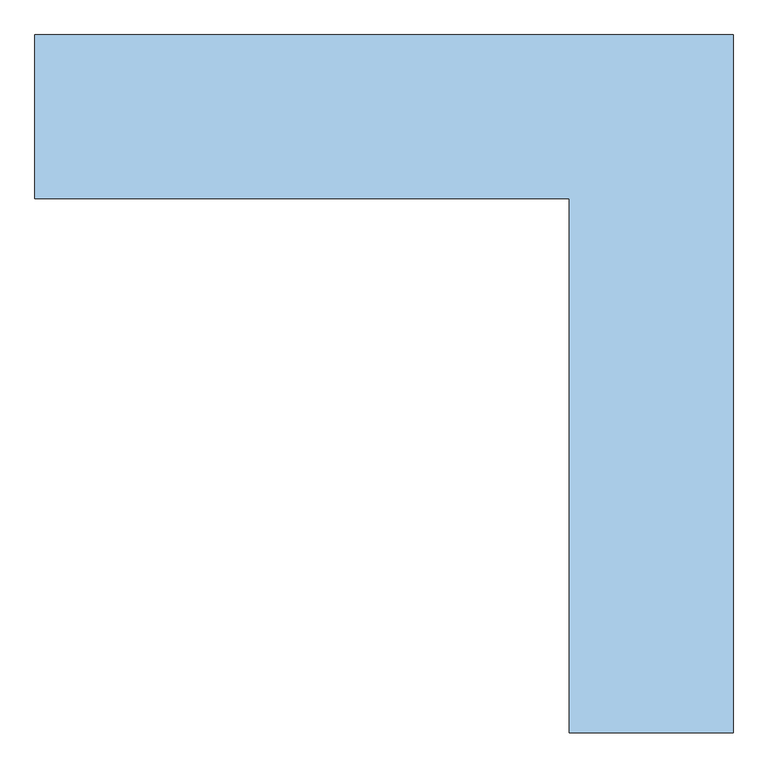
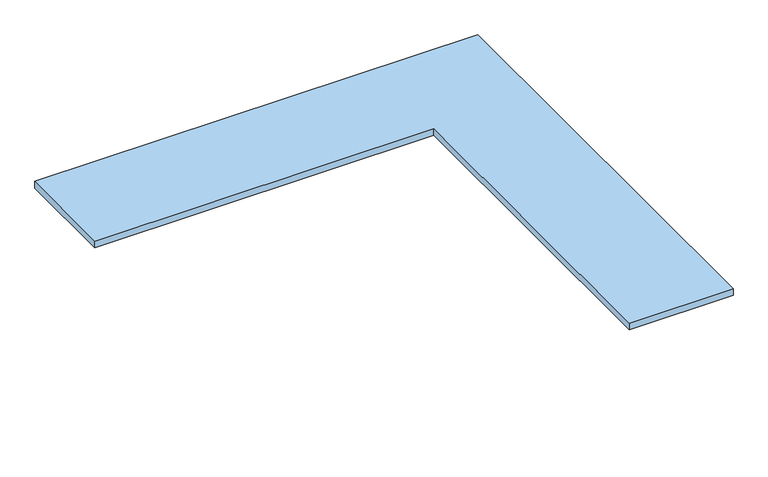
"""IFC4 building model written with IfcOpenShell, lengths in millimetres: window geometry, .CC_ND 300_PEDRA PEITORIL EM L : 1.26F x 1.26E x 0.30L."""

import ifcopenshell
import ifcopenshell.guid

model = None  # the IFC model being written
_history = None  # IfcOwnerHistory: only IFC2X3 demands one
_inside = {}  # id of a spatial element -> (the spatial element, [elements in it])
_under = {}  # id of a project, library or spatial element -> (it, [spatial elements below it])
_declared = {}  # id of a project -> (the project, [libraries it declares])
_typed = {}  # id of a type object -> (the type object, [elements of that type])
_made_of = {}  # id of a material, layer set ... -> (it, [elements and type objects made of it])


def new_model(schema):
    """Start an empty IFC model of exactly this schema.

    Asked for "IFC4X3", IfcOpenShell would pick the latest addendum, in which some entities
    have other attributes; the version numbers below select the first issue.
    IFC2X3 requires an IfcOwnerHistory on every rooted entity: one is made here for all.
    """
    global model, _history
    if schema == "IFC4X3":
        model = ifcopenshell.file(schema_version=(4, 3, 0, 0))
    else:
        model = ifcopenshell.file(schema=schema)
    _inside.clear()
    _under.clear()
    _declared.clear()
    _typed.clear()
    _made_of.clear()
    _history = None
    if model.schema == "IFC2X3":
        org = make("IfcOrganization", Name="unknown")
        user = make(
            "IfcPersonAndOrganization",
            ThePerson=make("IfcPerson", FamilyName="unknown"),
            TheOrganization=org,
        )
        app = make(
            "IfcApplication",
            ApplicationDeveloper=org,
            Version="unknown",
            ApplicationFullName="unknown",
            ApplicationIdentifier="unknown",
        )
        _history = make(
            "IfcOwnerHistory",
            OwningUser=user,
            OwningApplication=app,
            ChangeAction="ADDED",
            CreationDate=0,
        )
    return model


def make(cls, **values):
    """One entity of the class cls with the attributes given. An attribute that is None is left unset."""
    return model.create_entity(
        cls, **{name: value for name, value in values.items() if value is not None}
    )


def rooted(cls, **values):
    """An entity with a GlobalId (a new one), such as an element, a storey or a relation."""
    return make(cls, GlobalId=ifcopenshell.guid.new(), OwnerHistory=_history, **values)


def si_unit(unit_type, name, prefix=None):
    """IfcSIUnit, for example si_unit("LENGTHUNIT", "METRE", prefix="MILLI")."""
    return make("IfcSIUnit", UnitType=unit_type, Prefix=prefix, Name=name)


def assignment(units):
    """IfcUnitAssignment: the units of a project."""
    return None if units is None else make("IfcUnitAssignment", Units=units)


def point(xyz):
    """IfcCartesianPoint."""
    return None if xyz is None else make("IfcCartesianPoint", Coordinates=xyz)


def direction(xyz):
    """IfcDirection."""
    return None if xyz is None else make("IfcDirection", DirectionRatios=xyz)


def frame(location, z_axis=None, x_axis=None):
    """IfcAxis2Placement3D, a coordinate frame: its origin and axes. An axis left out is left unset."""
    return make(
        "IfcAxis2Placement3D",
        Location=point(location),
        Axis=direction(z_axis),
        RefDirection=direction(x_axis),
    )


def origin():
    """The frame at (0, 0, 0) with its axes left unset."""
    return frame((0.0, 0.0, 0.0))


def place(relative_to, where):
    """IfcLocalPlacement: puts the frame where relative to a parent placement (None: the world)."""
    return make(
        "IfcLocalPlacement", PlacementRelTo=relative_to, RelativePlacement=where
    )


def context(
    kind, dimensions, precision=None, world=None, true_north=None, identifier=None
):
    """IfcGeometricRepresentationContext, for example the 3D "Model" context."""
    return make(
        "IfcGeometricRepresentationContext",
        ContextIdentifier=identifier,
        ContextType=kind,
        CoordinateSpaceDimension=dimensions,
        Precision=precision,
        WorldCoordinateSystem=world,
        TrueNorth=true_north,
    )


def project(units=None, contexts=None):
    """IfcProject with its units and contexts."""
    return rooted(
        "IfcProject",
        Name="project",
        RepresentationContexts=contexts,
        UnitsInContext=assignment(units),
    )


def spatial(cls, under=None, at=None, **own):
    """A site, building, storey or space (cls), placed at a placement, below another one or the project."""
    s = rooted(cls, ObjectPlacement=at, **own)
    if under is not None:
        _under.setdefault(under.id(), (under, []))[1].append(s)
    return s


def polyline(points):
    """IfcPolyline through the points."""
    return make("IfcPolyline", Points=[point(p) for p in points])


def outline(outer, holes=None, kind="AREA"):
    """IfcArbitraryClosedProfileDef: a profile drawn as a closed curve; with holes, ...WithVoids."""
    if holes is None:
        return make("IfcArbitraryClosedProfileDef", ProfileType=kind, OuterCurve=outer)
    return make(
        "IfcArbitraryProfileDefWithVoids",
        ProfileType=kind,
        OuterCurve=outer,
        InnerCurves=holes,
    )


def extrude(swept, where, along, depth):
    """IfcExtrudedAreaSolid: the profile swept, set in the frame where, extruded along a direction by depth."""
    return make(
        "IfcExtrudedAreaSolid",
        SweptArea=swept,
        Position=where,
        ExtrudedDirection=direction(along),
        Depth=depth,
    )


def shape(context_of_items, identifier, shape_type, items):
    """IfcShapeRepresentation: the items that make up one representation, for example the "Body"."""
    return make(
        "IfcShapeRepresentation",
        ContextOfItems=context_of_items,
        RepresentationIdentifier=identifier,
        RepresentationType=shape_type,
        Items=items,
    )


def source(mapping_origin, context_of_items, identifier, shape_type, items):
    """IfcRepresentationMap: a shape defined once, which mapped items show again and again."""
    return make(
        "IfcRepresentationMap",
        MappingOrigin=mapping_origin,
        MappedRepresentation=shape(context_of_items, identifier, shape_type, items),
    )


def transform(
    local_origin,
    x_axis=None,
    y_axis=None,
    z_axis=None,
    scale=None,
    scale2=None,
    scale3=None,
    uniform=True,
):
    """IfcCartesianTransformationOperator3D, or its non-uniform kind. x_axis, y_axis, z_axis: its Axis1, 2, 3."""
    if uniform:
        return make(
            "IfcCartesianTransformationOperator3D",
            Axis1=direction(x_axis),
            Axis2=direction(y_axis),
            LocalOrigin=point(local_origin),
            Scale=scale,
            Axis3=direction(z_axis),
        )
    return make(
        "IfcCartesianTransformationOperator3DnonUniform",
        Axis1=direction(x_axis),
        Axis2=direction(y_axis),
        LocalOrigin=point(local_origin),
        Scale=scale,
        Axis3=direction(z_axis),
        Scale2=scale2,
        Scale3=scale3,
    )


def mapped(mapping_source, mapping_target):
    """IfcMappedItem: shows the shape of a source again, moved by a transform."""
    return make(
        "IfcMappedItem", MappingSource=mapping_source, MappingTarget=mapping_target
    )


def made_of(thing, what):
    """Note that an element or type object is made of a material, layer set ...; save() writes the relation."""
    if what is not None:
        _made_of.setdefault(what.id(), (what, []))[1].append(thing)
    return thing


def element(
    cls,
    number,
    at=None,
    inside=None,
    cuts=None,
    type_object=None,
    material=None,
    context=None,
    identifier="Body",
    shape_type=None,
    held_by="IfcProductDefinitionShape",
    body=None,
    shapes=None,
    **own,
):
    """One element of the class cls, such as IfcWall. Its Tag is "e" and its number.

    at: its placement. inside: the storey or other place that contains it. cuts: it is an
    opening in that element (IfcRelVoidsElement). A single representation is given by context,
    identifier, shape_type and body (its items); several are given by shapes. held_by: the class
    of the entity that holds the representations. save() writes the other relations.
    """
    e = rooted(cls, Tag="e%d" % number, ObjectPlacement=at, **own)
    if body is not None:
        shapes = [shape(context, identifier, shape_type, body)]
    if shapes is not None:
        e.Representation = make(held_by, Representations=shapes)
    if inside is not None:
        _inside.setdefault(inside.id(), (inside, []))[1].append(e)
    if cuts is not None:
        rooted(
            "IfcRelVoidsElement", RelatingBuildingElement=cuts, RelatedOpeningElement=e
        )
    if type_object is not None:
        _typed.setdefault(type_object.id(), (type_object, []))[1].append(e)
    return made_of(e, material)


def aggregate(whole, parts):
    """IfcRelAggregates: a whole, such as a stair, and the parts it consists of."""
    return rooted("IfcRelAggregates", RelatingObject=whole, RelatedObjects=parts)


def save(model, path):
    """Write the relations noted so far, then the file.

    IfcRelAggregates (storeys below a building ...), IfcRelContainedInSpatialStructure (elements
    in a storey), IfcRelDefinesByType, IfcRelAssociatesMaterial and IfcRelDeclares: one each for
    every whole, place, type object, material and project.
    """
    for whole, parts in _under.values():
        aggregate(whole, parts)
    for where, things in _inside.values():
        rooted(
            "IfcRelContainedInSpatialStructure",
            RelatedElements=things,
            RelatingStructure=where,
        )
    for kind, things in _typed.values():
        rooted("IfcRelDefinesByType", RelatedObjects=things, RelatingType=kind)
    for what, things in _made_of.values():
        rooted("IfcRelAssociatesMaterial", RelatedObjects=things, RelatingMaterial=what)
    for by, libraries in _declared.values():
        rooted("IfcRelDeclares", RelatingContext=by, RelatedDefinitions=libraries)
    model.write(path)


def window_94eaf2cf(model_context):
    return source(origin(), model_context, "Body", "SweptSolid", [
        extrude(outline(polyline([(-615.0, -147.5), (-615.0, 148.0), (645.0, 148.0), (645.0, -1112.0), (349.5, -1112.0), (349.5, -147.5), (-615.0, -147.5)])), frame((0.0, 0.0, 900.0), z_axis=(0.0, 0.0, 1.0), x_axis=(1.0, 0.0, 0.0)), (0.0, 0.0, 1.0), 20.0),
    ])


if __name__ == "__main__":
    model = new_model("IFC4")
    model_context = context("Model", 3, world=origin())
    ifc_project = project(units=[si_unit("LENGTHUNIT", "METRE", prefix="MILLI")], contexts=[model_context])
    site = spatial("IfcSite", under=ifc_project)
    building = spatial("IfcBuilding", under=site)
    placement = place(None, origin())
    window_shape = window_94eaf2cf(model_context)
    element("IfcWindow", 1, ObjectType=".CC_ND 300_PEDRA PEITORIL EM L : 1.26F x 1.26E x 0.30L", at=placement, inside=building, context=model_context, shape_type="MappedRepresentation", body=[
        mapped(window_shape, transform((0.0, 0.0, 0.0), x_axis=(1.0, 0.0, 0.0), y_axis=(0.0, 1.0, 0.0), z_axis=(0.0, 0.0, 1.0))),
    ])
    save(model, "model.ifc")

# Revit data of these elements
# Type ".CC_ND 300_PEDRA PEITORIL EM L : 1.26F x 1.26E x 0.30L"
#   Type Mark = "73"
#   Largura da pedra da frente [instance default] = 0.26 m
#   Largura da pedra da esquerda [instance default] = 0.26 m
#   Extensão esquerda interna [instance default] = 0.03 m
#   Extensão esquerda externa [instance default] = 0.03 m
#   Comprimento Esquerda = 0.9645 m
#   Extensão frente interna [instance default] = 0.03 m
#   Extensão frente externa [instance default] = 0.03 m
#   Espessura peitoril = 0.02 m
#   Espessura da parede [instance default] = 0.20 m
#   Comprimento da pedra [instance default] = 2.1945 m
#   Comprimento Frente = 1.23 m
#   Altura-padrão do peitoril [instance default] = 0.90 m
#   Pedra do peitoril = .GRANITO_BRANCO_ITAUNAS
#   Rough Width = 0
#   Rough Height = 0
#   Height = 0
#   Wall Closure = (empty or 0)
#   Width = 0
# Element 1 (IfcWindow, ".CC_ND 300_PEDRA PEITORIL EM L : 1.26F x 1.26E x 0.30L")
#   Largura da pedra da frente = 0.2955 m
#   Largura da pedra da esquerda = 0.2955 m
#   Extensão esquerda interna = 0.0295 m
#   Extensão frente interna = 0.0295 m
#   Espessura da parede = 0.236 m
#   Materials on its faces: ".GRANITO_BRANCO_ITAUNAS"
# Materials
#   ".GRANITO_BRANCO_ITAUNAS": class ".CC_PEDRA REVEST.", colour RGB 202 195 174, transparency 0, Description = "Revestimento em granito", Cost = 0
